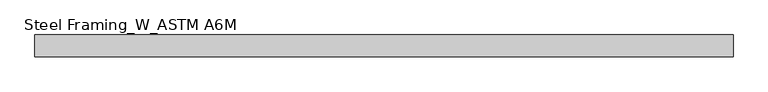
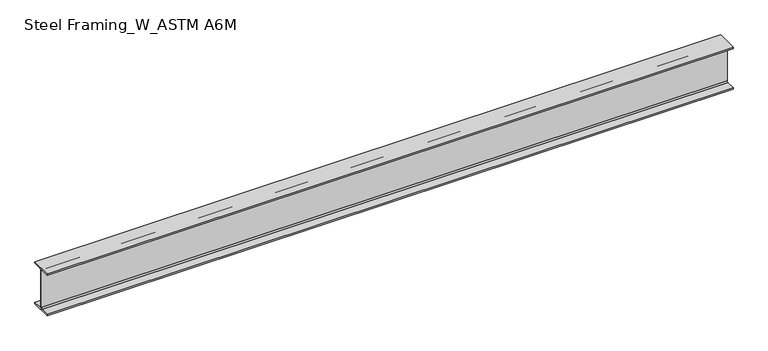
"""IFC4 building model written with IfcOpenShell, lengths in millimetres: beam geometry, Steel Framing_W_ASTM A6M : H_SB_AR_S02_W360x51_RG1."""

from ifc_helpers import new_model, si_unit, point, frame, frame_2d, origin, place, context, project, spatial, polyline, circle_curve, trimmed, segment, composite_curve, outline, extrude, source, transform, mapped, element, save


def steel_framing_w_astm_a6m_020ad02a(model_context):
    return source(origin(), model_context, "Body", "SweptSolid", [
        extrude(outline(composite_curve([segment(polyline([(85.5, -166.4), (85.5, -178.0), (-85.5, -178.0), (-85.5, -166.4), (-13.72, -166.4)]), True, "CONTINUOUS"), segment(trimmed(circle_curve(frame_2d((-13.72, -156.3)), 10.1), [point((-13.72, -166.4))], [point((-3.62, -156.3))], True, "CARTESIAN"), True, "CONTINUOUS"), segment(polyline([(-3.62, -156.3), (-3.62, 156.3)]), True, "CONTINUOUS"), segment(trimmed(circle_curve(frame_2d((-13.72, 156.3)), 10.1), [point((-3.62, 156.3))], [point((-13.72, 166.4))], True, "CARTESIAN"), True, "CONTINUOUS"), segment(polyline([(-13.72, 166.4), (-85.5, 166.4), (-85.5, 178.0), (85.5, 178.0), (85.5, 166.4), (13.72, 166.4)]), True, "CONTINUOUS"), segment(trimmed(circle_curve(frame_2d((13.72, 156.3)), 10.1), [point((13.72, 166.4))], [point((3.62, 156.3))], True, "CARTESIAN"), True, "CONTINUOUS"), segment(polyline([(3.62, 156.3), (3.62, -156.3)]), True, "CONTINUOUS"), segment(trimmed(circle_curve(frame_2d((13.72, -156.3)), 10.1), [point((3.62, -156.3))], [point((13.72, -166.4))], True, "CARTESIAN"), True, "CONTINUOUS"), segment(polyline([(13.72, -166.4), (85.5, -166.4)]), True, "CONTINUOUS")], self_intersect=False)), frame((-2731.95, 0.0, 0.0), z_axis=(1.0, 0.0, 0.0), x_axis=(0.0, 1.0, 0.0)), (0.0, 0.0, 1.0), 5501.8),
    ])


if __name__ == "__main__":
    model = new_model("IFC4")
    model_context = context("Model", 3, world=origin())
    ifc_project = project(units=[si_unit("LENGTHUNIT", "METRE", prefix="MILLI")], contexts=[model_context])
    site = spatial("IfcSite", under=ifc_project)
    building = spatial("IfcBuilding", under=site)
    placement = place(None, origin())
    steel_framing_w_astm_a6m_shape = steel_framing_w_astm_a6m_020ad02a(model_context)
    element("IfcBeam", 1, ObjectType="Steel Framing_W_ASTM A6M : H_SB_AR_S02_W360x51_RG1", at=placement, inside=building, context=model_context, shape_type="MappedRepresentation", body=[
        mapped(steel_framing_w_astm_a6m_shape, transform((0.0, 0.0, 0.0), x_axis=(1.0, 0.0, 0.0), y_axis=(0.0, 1.0, 0.0), z_axis=(0.0, 0.0, 1.0))),
    ])
    save(model, "model.ifc")

# Revit data of these elements
# Type "Steel Framing_W_ASTM A6M : H_SB_AR_S02_W360x51_RG1"
#   Section Name Key = "W14x34"
#   Width = 17.1 cm
#   Web Thickness = 0.724 cm
#   Web Fillet = 1.01 cm
#   Warping Constant = 287000.0 cm⁶
#   Torsional Moment of Inertia = 23.70 cm⁴
#   Section Area = 64.5 cm²
#   Plastic Modulus weak axis = 174.0 cm³
#   Plastic Modulus strong axis = 895.0 cm³
#   Perimeter = 1.36 m²/m
#   Nominal Weight = 51.00 kgf/m
#   Moment of Inertia weak axis = 970.00 cm⁴
#   Moment of Inertia strong axis = 14200.00 cm⁴
#   Height = 35.6 cm
#   Flange Thickness = 1.16 cm
#   Elastic Modulus weak axis = 113.0 cm³
#   Elastic Modulus strong axis = 796.0 cm³
#   Centroid Vertical = 17.8 cm
#   Centroid Horizontal = 8.55 cm
#   Length [instance default] = 1500 mm
#   Structural Material [instance default] = Steel, 45-345
#   Bolt Spacing = 0
#   Assembly Code = ""
# Element 1 (IfcBeam, "Steel Framing_W_ASTM A6M : H_SB_AR_S02_W360x51_RG1")
#   Materials on its faces: "Steel, 45-345"
# Materials
#   "Steel, 45-345": class "Metal", colour RGB 189 187 185, transparency 0, Description = "Steel 345 MPa", Cost = 0
